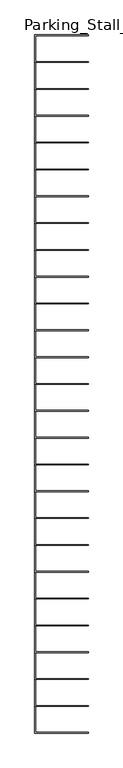
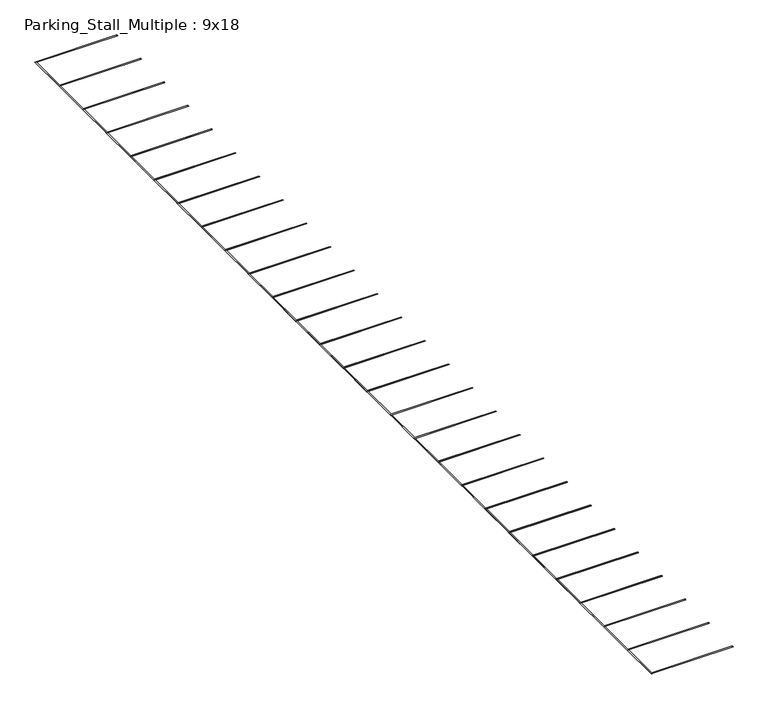
"""IFC4 building model written with IfcOpenShell, lengths in millimetres: proxy geometry, Parking_Stall_Multiple : 9x18."""

from ifc_helpers import new_model, si_unit, origin, origin_with_axes, place, context, project, spatial, polyline, outline, extrude, source, transform, mapped, element, save


def parking_stall_multiple_9x18_b666618d(model_context):
    return source(origin(), model_context, "Body", "SweptSolid", [
        extrude(outline(polyline([(5486.4, 68580.0), (0.0, 68580.0), (0.0, 71399.4), (5486.4, 71399.4), (5486.4, 71323.2), (76.2, 71323.2), (76.2, 68656.2), (5486.4, 68656.2), (5486.4, 68580.0)])), origin_with_axes(), (0.0, 0.0, 1.0), 6.35),
        extrude(outline(polyline([(5486.4, 65836.8), (0.0, 65836.8), (0.0, 68656.2), (5486.4, 68656.2), (5486.4, 68580.0), (76.2, 68580.0), (76.2, 65913.0), (5486.4, 65913.0), (5486.4, 65836.8)])), origin_with_axes(), (0.0, 0.0, 1.0), 6.35),
        extrude(outline(polyline([(5486.4, 63093.6), (0.0, 63093.6), (0.0, 65913.0), (5486.4, 65913.0), (5486.4, 65836.8), (76.2, 65836.8), (76.2, 63169.8), (5486.4, 63169.8), (5486.4, 63093.6)])), origin_with_axes(), (0.0, 0.0, 1.0), 6.35),
        extrude(outline(polyline([(5486.4, 60350.4), (0.0, 60350.4), (0.0, 63169.8), (5486.4, 63169.8), (5486.4, 63093.6), (76.2, 63093.6), (76.2, 60426.6), (5486.4, 60426.6), (5486.4, 60350.4)])), origin_with_axes(), (0.0, 0.0, 1.0), 6.35),
        extrude(outline(polyline([(5486.4, 57607.2), (0.0, 57607.2), (0.0, 60426.6), (5486.4, 60426.6), (5486.4, 60350.4), (76.2, 60350.4), (76.2, 57683.4), (5486.4, 57683.4), (5486.4, 57607.2)])), origin_with_axes(), (0.0, 0.0, 1.0), 6.35),
        extrude(outline(polyline([(5486.4, 54864.0), (0.0, 54864.0), (0.0, 57683.4), (5486.4, 57683.4), (5486.4, 57607.2), (76.2, 57607.2), (76.2, 54940.2), (5486.4, 54940.2), (5486.4, 54864.0)])), origin_with_axes(), (0.0, 0.0, 1.0), 6.35),
        extrude(outline(polyline([(5486.4, 52120.8), (0.0, 52120.8), (0.0, 54940.2), (5486.4, 54940.2), (5486.4, 54864.0), (76.2, 54864.0), (76.2, 52197.0), (5486.4, 52197.0), (5486.4, 52120.8)])), origin_with_axes(), (0.0, 0.0, 1.0), 6.35),
        extrude(outline(polyline([(5486.4, 49377.6), (0.0, 49377.6), (0.0, 52197.0), (5486.4, 52197.0), (5486.4, 52120.8), (76.2, 52120.8), (76.2, 49453.8), (5486.4, 49453.8), (5486.4, 49377.6)])), origin_with_axes(), (0.0, 0.0, 1.0), 6.35),
        extrude(outline(polyline([(5486.4, 46634.4), (0.0, 46634.4), (0.0, 49453.8), (5486.4, 49453.8), (5486.4, 49377.6), (76.2, 49377.6), (76.2, 46710.6), (5486.4, 46710.6), (5486.4, 46634.4)])), origin_with_axes(), (0.0, 0.0, 1.0), 6.35),
        extrude(outline(polyline([(5486.4, 43891.2), (0.0, 43891.2), (0.0, 46710.6), (5486.4, 46710.6), (5486.4, 46634.4), (76.2, 46634.4), (76.2, 43967.4), (5486.4, 43967.4), (5486.4, 43891.2)])), origin_with_axes(), (0.0, 0.0, 1.0), 6.35),
        extrude(outline(polyline([(5486.4, 41148.0), (0.0, 41148.0), (0.0, 43967.4), (5486.4, 43967.4), (5486.4, 43891.2), (76.2, 43891.2), (76.2, 41224.2), (5486.4, 41224.2), (5486.4, 41148.0)])), origin_with_axes(), (0.0, 0.0, 1.0), 6.35),
        extrude(outline(polyline([(5486.4, 38404.8), (0.0, 38404.8), (0.0, 41224.2), (5486.4, 41224.2), (5486.4, 41148.0), (76.2, 41148.0), (76.2, 38481.0), (5486.4, 38481.0), (5486.4, 38404.8)])), origin_with_axes(), (0.0, 0.0, 1.0), 6.35),
        extrude(outline(polyline([(5486.4, 35661.6), (0.0, 35661.6), (0.0, 38481.0), (5486.4, 38481.0), (5486.4, 38404.8), (76.2, 38404.8), (76.2, 35737.8), (5486.4, 35737.8), (5486.4, 35661.6)])), origin_with_axes(), (0.0, 0.0, 1.0), 6.35),
        extrude(outline(polyline([(5486.4, 32918.4), (0.0, 32918.4), (0.0, 35737.8), (5486.4, 35737.8), (5486.4, 35661.6), (76.2, 35661.6), (76.2, 32994.6), (5486.4, 32994.6), (5486.4, 32918.4)])), origin_with_axes(), (0.0, 0.0, 1.0), 6.35),
        extrude(outline(polyline([(5486.4, 30175.2), (0.0, 30175.2), (0.0, 32994.6), (5486.4, 32994.6), (5486.4, 32918.4), (76.2, 32918.4), (76.2, 30251.4), (5486.4, 30251.4), (5486.4, 30175.2)])), origin_with_axes(), (0.0, 0.0, 1.0), 6.35),
        extrude(outline(polyline([(5486.4, 27432.0), (0.0, 27432.0), (0.0, 30251.4), (5486.4, 30251.4), (5486.4, 30175.2), (76.2, 30175.2), (76.2, 27508.2), (5486.4, 27508.2), (5486.4, 27432.0)])), origin_with_axes(), (0.0, 0.0, 1.0), 6.35),
        extrude(outline(polyline([(5486.4, 24688.8), (0.0, 24688.8), (0.0, 27508.2), (5486.4, 27508.2), (5486.4, 27432.0), (76.2, 27432.0), (76.2, 24765.0), (5486.4, 24765.0), (5486.4, 24688.8)])), origin_with_axes(), (0.0, 0.0, 1.0), 6.35),
        extrude(outline(polyline([(5486.4, 21945.6), (0.0, 21945.6), (0.0, 24765.0), (5486.4, 24765.0), (5486.4, 24688.8), (76.2, 24688.8), (76.2, 22021.8), (5486.4, 22021.8), (5486.4, 21945.6)])), origin_with_axes(), (0.0, 0.0, 1.0), 6.35),
        extrude(outline(polyline([(5486.4, 19202.4), (0.0, 19202.4), (0.0, 22021.8), (5486.4, 22021.8), (5486.4, 21945.6), (76.2, 21945.6), (76.2, 19278.6), (5486.4, 19278.6), (5486.4, 19202.4)])), origin_with_axes(), (0.0, 0.0, 1.0), 6.35),
        extrude(outline(polyline([(5486.4, 16459.2), (0.0, 16459.2), (0.0, 19278.6), (5486.4, 19278.6), (5486.4, 19202.4), (76.2, 19202.4), (76.2, 16535.4), (5486.4, 16535.4), (5486.4, 16459.2)])), origin_with_axes(), (0.0, 0.0, 1.0), 6.35),
        extrude(outline(polyline([(5486.4, 13716.0), (0.0, 13716.0), (0.0, 16535.4), (5486.4, 16535.4), (5486.4, 16459.2), (76.2, 16459.2), (76.2, 13792.2), (5486.4, 13792.2), (5486.4, 13716.0)])), origin_with_axes(), (0.0, 0.0, 1.0), 6.35),
        extrude(outline(polyline([(5486.4, 10972.8), (0.0, 10972.8), (0.0, 13792.2), (5486.4, 13792.2), (5486.4, 13716.0), (76.2, 13716.0), (76.2, 11049.0), (5486.4, 11049.0), (5486.4, 10972.8)])), origin_with_axes(), (0.0, 0.0, 1.0), 6.35),
        extrude(outline(polyline([(5486.4, 8229.6), (0.0, 8229.6), (0.0, 11049.0), (5486.4, 11049.0), (5486.4, 10972.8), (76.2, 10972.8), (76.2, 8305.8), (5486.4, 8305.8), (5486.4, 8229.6)])), origin_with_axes(), (0.0, 0.0, 1.0), 6.35),
        extrude(outline(polyline([(5486.4, 5486.4), (0.0, 5486.4), (0.0, 8305.8), (5486.4, 8305.8), (5486.4, 8229.6), (76.2, 8229.6), (76.2, 5562.6), (5486.4, 5562.6), (5486.4, 5486.4)])), origin_with_axes(), (0.0, 0.0, 1.0), 6.35),
        extrude(outline(polyline([(5486.4, 2743.2), (0.0, 2743.2), (0.0, 5562.6), (5486.4, 5562.6), (5486.4, 5486.4), (76.2, 5486.4), (76.2, 2819.4), (5486.4, 2819.4), (5486.4, 2743.2)])), origin_with_axes(), (0.0, 0.0, 1.0), 6.35),
        extrude(outline(polyline([(5486.4, 0.0), (0.0, 0.0), (0.0, 2819.4), (5486.4, 2819.4), (5486.4, 2743.2), (76.2, 2743.2), (76.2, 76.2), (5486.4, 76.2), (5486.4, 0.0)])), origin_with_axes(), (0.0, 0.0, 1.0), 6.35),
    ])


if __name__ == "__main__":
    model = new_model("IFC4")
    model_context = context("Model", 3, world=origin())
    ifc_project = project(units=[si_unit("LENGTHUNIT", "METRE", prefix="MILLI")], contexts=[model_context])
    site = spatial("IfcSite", under=ifc_project)
    building = spatial("IfcBuilding", under=site)
    placement = place(None, origin())
    parking_stall_multiple_9x18_shape = parking_stall_multiple_9x18_b666618d(model_context)
    element("IfcBuildingElementProxy", 1, Name="Parking_Stall_Multiple : 9x18", ObjectType="Parking_Stall_Multiple : 9x18", at=placement, inside=building, context=model_context, shape_type="MappedRepresentation", body=[
        mapped(parking_stall_multiple_9x18_shape, transform((0.0, 0.0, 0.0), x_axis=(1.0, 0.0, 0.0), y_axis=(0.0, 1.0, 0.0), z_axis=(0.0, 0.0, 1.0))),
    ])
    save(model, "model.ifc")

# Revit data of these elements
# Type "Parking_Stall_Multiple : 9x18"
#   Parking_Width_M = 9' - 0"
#   Parking_Run_Length [instance default] = 65' - 0"
#   Parking_Line_Width = 0' - 3"
#   Parking_Length_M = 18' - 0"
#   Single_Parking_Visibility [instance default] = no
#   Parking_ADA_Symbol = no
#   ParkingUnitsArray [instance default] = 7
#   ParkingUnits [instance default] = 7
#   Multiple_Parking_Visibility [instance default] = yes
#   Parking_Line_Material = none
# Element 1 (IfcBuildingElementProxy, "Parking_Stall_Multiple : 9x18")
#   Parking_Run_Length = 237' - 6.80354"
#   ParkingUnitsArray = 26
#   ParkingUnits = 26
